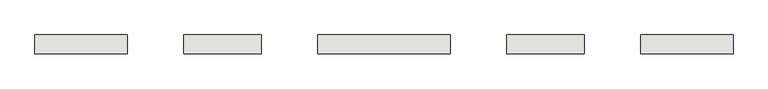
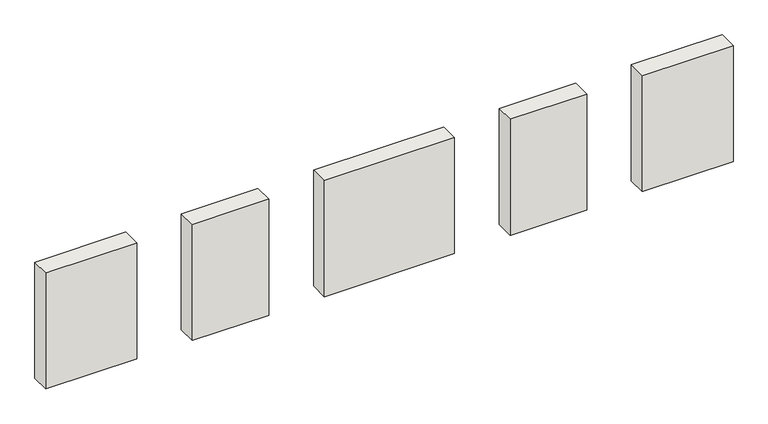
"""IFC4 building model written with IfcOpenShell, lengths in millimetres: wall geometry, 0_3d."""

from ifc_helpers import new_model, si_unit, origin, origin_with_axes, place, context, project, spatial, polyline, outline, extrude, source, transform, mapped, element, save


def wall_25e8281b(model_context):
    return source(origin(), model_context, "Body", "SweptSolid", [
        extrude(outline(polyline([(1850.0, 380.0), (1850.0, 0.0), (0.0, 0.0), (0.0, 380.0), (1850.0, 380.0)])), origin_with_axes(), (0.0, 0.0, 1.0), 2500.0),
        extrude(outline(polyline([(2985.0, 0.0), (2985.0, 380.0), (4540.0, 380.0), (4540.0, 0.0), (2985.0, 0.0)])), origin_with_axes(), (0.0, 0.0, 1.0), 2500.0),
        extrude(outline(polyline([(5675.0, 0.0), (5675.0, 380.0), (8325.0, 380.0), (8325.0, 0.0), (5675.0, 0.0)])), origin_with_axes(), (0.0, 0.0, 1.0), 2500.0),
        extrude(outline(polyline([(11015.0, 380.0), (11015.0, 0.0), (9460.0, 0.0), (9460.0, 380.0), (11015.0, 380.0)])), origin_with_axes(), (0.0, 0.0, 1.0), 2500.0),
        extrude(outline(polyline([(12150.0, 0.0), (12150.0, 380.0), (14000.0, 380.0), (14000.0, 0.0), (12150.0, 0.0)])), origin_with_axes(), (0.0, 0.0, 1.0), 2500.0),
    ])


if __name__ == "__main__":
    model = new_model("IFC4")
    model_context = context("Model", 3, world=origin())
    ifc_project = project(units=[si_unit("LENGTHUNIT", "METRE", prefix="MILLI")], contexts=[model_context])
    site = spatial("IfcSite", under=ifc_project)
    building = spatial("IfcBuilding", under=site)
    placement = place(None, origin())
    wall_shape = wall_25e8281b(model_context)
    element("IfcWall", 1, ObjectType="0_3d", at=placement, inside=building, context=model_context, shape_type="MappedRepresentation", body=[
        mapped(wall_shape, transform((0.0, 0.0, 0.0), x_axis=(1.0, 0.0, 0.0), y_axis=(0.0, 1.0, 0.0), z_axis=(0.0, 0.0, 1.0))),
    ])
    save(model, "model.ifc")

# Revit data of these elements
# Element 1 (IfcWall, "0_3d")
#   Materials on its faces: "holzschalung"
# Materials
#   "holzschalung": class "Unassigned", colour RGB 128 128 128, transparency 0
